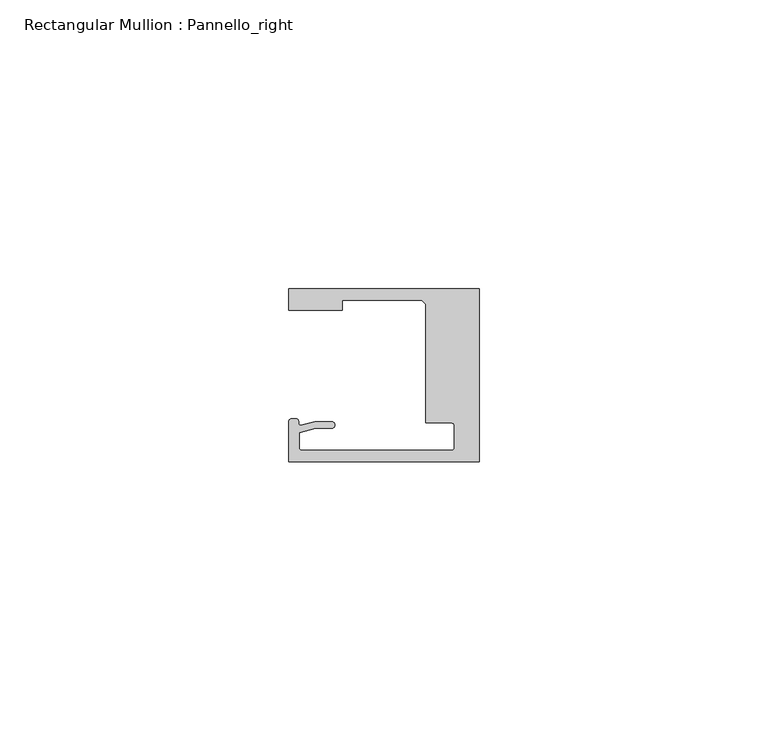
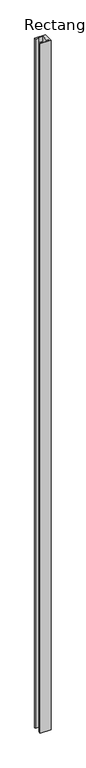
"""IFC4 building model written with IfcOpenShell, lengths in millimetres: member geometry, Rectangular Mullion : Pannello_right."""

from ifc_helpers import new_model, si_unit, frame, origin, place, context, project, spatial, polyline, circle_curve, source, transform, mapped, element, save
from ifc_brep_helpers import plane_surface, cylinder_surface, revolved_surface, extruded_surface, spline_curve, advanced_brep


def rectangular_mullion_pannello_right_fd8d7534(model_context):
    return source(origin(), model_context, "Body", "AdvancedBrep", [
        advanced_brep(
        [(-33.0, 15.0, 0.0), (-33.0, 11.3000004, 0.0), (-23.700041, 11.3000004, 0.0), (-23.700041, 13.0000004, 0.0), (-10.0000103, 13.0000004, 0.0), (-9.2999726, 12.2999849, 0.0), (-9.2999726, -8.2500595, 0.0), (-4.7999726, -8.2500595, 0.0), (-4.2999726, -8.7500595, 0.0), (-4.2999726, -12.50001, 0.0), (-4.7999726, -13.00001, 0.0), (-30.69998, -13.00001, 0.0), (-31.19998, -12.50001, 0.0), (-31.19998, -9.9657591, 0.0), (-28.3419477, -9.1999523, 0.0), (-25.59998, -9.1999523, 0.0), (-25.59998, -7.9999523, 0.0), (-28.4999305, -7.9999523, 0.0), (-30.9223017, -8.6490241, 0.0), (-33.0000135, -8.0000472, 0.0), (-33.0000135, -15.0, 0.0), (0.0, -15.0, 0.0), (0.0, 15.0, 0.0), (-33.0, 15.0, -2260.0), (0.0, 15.0, -2260.0), (0.0, -15.0, -2260.0), (-33.0000135, -15.0, -2260.0), (-33.0000135, -8.0000472, -2260.0), (-30.9223017, -8.6490241, -2260.0), (-28.4999305, -7.9999523, -2260.0), (-25.59998, -7.9999523, -2260.0), (-25.59998, -9.1999523, -2260.0), (-28.3419477, -9.1999523, -2260.0), (-31.19998, -9.9657591, -2260.0), (-31.19998, -12.50001, -2260.0), (-30.69998, -13.00001, -2260.0), (-4.7999726, -13.00001, -2260.0), (-4.2999726, -12.50001, -2260.0), (-4.2999726, -8.7500595, -2260.0), (-4.7999726, -8.2500595, -2260.0), (-9.2999726, -8.2500595, -2260.0), (-9.2999726, 12.2999849, -2260.0), (-10.0000103, 13.0000004, -2260.0), (-23.700041, 13.0000004, -2260.0), (-23.700041, 11.3000004, -2260.0), (-33.0, 11.3000004, -2260.0)],
        [
            (0, 1),
            (1, 2),
            (2, 3),
            (3, 4),
            (4, 5),
            (5, 6),
            (6, 7),
            (7, 8, circle_curve(frame((-4.7999726, -8.7500595, 0.0), z_axis=(0.0, 0.0, -1.0), x_axis=(0.0, 1.0, 0.0)), 0.5)),
            (8, 9),
            (9, 10, circle_curve(frame((-4.7999726, -12.50001, 0.0), z_axis=(0.0, 0.0, -1.0), x_axis=(1.0, 0.0, 0.0)), 0.5)),
            (10, 11),
            (11, 12, circle_curve(frame((-30.69998, -12.50001, 0.0), z_axis=(0.0, 0.0, -1.0), x_axis=(0.0, -1.0, 0.0)), 0.5)),
            (12, 13),
            (13, 14),
            (14, 15),
            (15, 16, circle_curve(frame((-25.59998, -8.5999523, 0.0), z_axis=(0.0, 0.0, 1.0), x_axis=(0.0, -1.0, 0.0)), 0.6)),
            (16, 17),
            (17, 18),
            (18, 19, spline_curve(3, [(-30.9223017, -8.6490241, 0.0), (-31.312054066, -8.717747958, 0.0), (-31.298563602, -8.366228555, 0.0), (-31.305645054, -7.690065204, 0.0), (-31.357433266, -7.563996614, 0.0), (-32.262327879, -7.456527435, 0.0), (-33.0000135, -7.457047519, 0.0), (-33.0000135, -8.0000472, 0.0)], [4, 2, 2, 4], [0.0, 0.001840817752199412, 0.004996616814974408, 0.007702013405570312])),
            (19, 20),
            (20, 21),
            (21, 22),
            (22, 0),
            (23, 24),
            (24, 25),
            (25, 26),
            (26, 27),
            (27, 28, spline_curve(3, [(-33.0000135, -8.0000472, -2260.0), (-33.0000135, -7.457047519, -2260.0), (-32.262327879, -7.456527435, -2260.0), (-31.357433266, -7.563996614, -2260.0), (-31.305645054, -7.690065204, -2260.0), (-31.298563602, -8.366228555, -2260.0), (-31.312054066, -8.717747958, -2260.0), (-30.9223017, -8.6490241, -2260.0)], [4, 2, 2, 4], [0.0, 0.0027053965905959043, 0.0058611956533709, 0.007702013405570312])),
            (28, 29),
            (29, 30),
            (30, 31, circle_curve(frame((-25.59998, -8.5999523, -2260.0), z_axis=(0.0, 0.0, -1.0), x_axis=(0.0, -1.0, 0.0)), 0.6)),
            (31, 32),
            (32, 33),
            (33, 34),
            (34, 35, circle_curve(frame((-30.69998, -12.50001, -2260.0), z_axis=(0.0, 0.0, 1.0), x_axis=(0.0, -1.0, 0.0)), 0.5)),
            (35, 36),
            (36, 37, circle_curve(frame((-4.7999726, -12.50001, -2260.0), z_axis=(0.0, 0.0, 1.0), x_axis=(1.0, 0.0, 0.0)), 0.5)),
            (37, 38),
            (38, 39, circle_curve(frame((-4.7999726, -8.7500595, -2260.0), z_axis=(0.0, 0.0, 1.0), x_axis=(0.0, 1.0, 0.0)), 0.5)),
            (39, 40),
            (40, 41),
            (41, 42),
            (42, 43),
            (43, 44),
            (44, 45),
            (45, 23),
            (0, 23),
            (45, 1),
            (44, 2),
            (43, 3),
            (42, 4),
            (41, 5),
            (40, 6),
            (39, 7),
            (38, 8),
            (37, 9),
            (36, 10),
            (35, 11),
            (34, 12),
            (33, 13),
            (32, 14),
            (31, 15),
            (30, 16),
            (29, 17),
            (28, 18),
            (27, 19),
            (26, 20),
            (25, 21),
            (24, 22),
        ],
        [
            plane_surface(frame((0.0, -36.2491502, 0.0), z_axis=(0.0, 0.0, 1.0), x_axis=(-1.0, 0.0, 0.0))),
            plane_surface(frame((0.0, -36.2491502, -2260.0), z_axis=(0.0, 0.0, -1.0), x_axis=(-1.0, 0.0, 0.0))),
            plane_surface(frame((-33.0, 15.0, 0.0), z_axis=(-1.0, 0.0, 0.0), x_axis=(0.0, 0.0, -1.0))),
            plane_surface(frame((-33.0, 11.3000004, 0.0), z_axis=(0.0, -1.0, 0.0), x_axis=(0.0, 0.0, -1.0))),
            plane_surface(frame((-23.700041, 11.3000004, 0.0), z_axis=(1.0, 0.0, 0.0), x_axis=(0.0, 0.0, -1.0))),
            plane_surface(frame((-23.700041, 13.0000004, 0.0), z_axis=(0.0, -1.0, 0.0), x_axis=(0.0, 0.0, -1.0))),
            plane_surface(frame((-10.0000103, 13.0000004, 0.0), z_axis=(-0.7070955486278075, -0.7071180135668587, 0.0), x_axis=(0.0, 0.0, -1.0))),
            plane_surface(frame((-9.2999726, 12.2999849, 0.0), z_axis=(-1.0, 0.0, 0.0), x_axis=(0.0, 0.0, -1.0))),
            plane_surface(frame((-9.2999726, -8.2500595, 0.0), z_axis=(0.0, -1.0, 0.0), x_axis=(0.0, 0.0, -1.0))),
            revolved_surface(polyline([(-4.7999726, -8.2500595, -2260.0), (-4.7999726, -8.2500595, 0.0)]), (-4.7999726, -8.7500595, 0.0), (0.0, 0.0, -1.0)),
            plane_surface(frame((-4.2999726, -8.7500595, 0.0), z_axis=(-1.0, 0.0, 0.0), x_axis=(0.0, 0.0, -1.0))),
            revolved_surface(polyline([(-4.2999726, -12.50001, -2260.0), (-4.2999726, -12.50001, 0.0)]), (-4.7999726, -12.50001, 0.0), (0.0, 0.0, -1.0)),
            plane_surface(frame((-4.7999726, -13.00001, 0.0), z_axis=(0.0, 1.0, 0.0), x_axis=(0.0, 0.0, -1.0))),
            revolved_surface(polyline([(-30.69998, -13.00001, -2260.0), (-30.69998, -13.00001, 0.0)]), (-30.69998, -12.50001, 0.0), (0.0, 0.0, -1.0)),
            plane_surface(frame((-31.19998, -12.50001, 0.0), z_axis=(1.0, 0.0, 0.0), x_axis=(0.0, 0.0, -1.0))),
            plane_surface(frame((-31.19998, -9.9657591, 0.0), z_axis=(0.2588188320428738, -0.9659258833782035, 0.0), x_axis=(0.0, 0.0, -1.0))),
            plane_surface(frame((-28.3419477, -9.1999523, 0.0), z_axis=(0.0, -1.0, 0.0), x_axis=(0.0, 0.0, -1.0))),
            cylinder_surface(frame((-25.59998, -8.5999523, 0.0), z_axis=(0.0, 0.0, 1.0), x_axis=(0.0, -1.0, 0.0)), 0.6),
            plane_surface(frame((-25.59998, -7.9999523, 0.0), z_axis=(0.0, 1.0, 0.0), x_axis=(0.0, 0.0, -1.0))),
            plane_surface(frame((-28.4999305, -7.9999523, 0.0), z_axis=(-0.2588188320019168, 0.965925883389178, 0.0), x_axis=(0.0, 0.0, -1.0))),
            extruded_surface(spline_curve(3, [(-30.9223017, -8.6490241, -2260.0), (-31.312054066, -8.717747958, -2260.0), (-31.298563602, -8.366228555, -2260.0), (-31.305645054, -7.690065204, -2260.0), (-31.357433266, -7.563996614, -2260.0), (-32.262327879, -7.456527435, -2260.0), (-33.0000135, -7.457047519, -2260.0), (-33.0000135, -8.0000472, -2260.0)], [4, 2, 2, 4], [0.0, 0.001840817752199412, 0.004996616814974408, 0.007702013405570312]), (0.0, 0.0, 2260.0), 2260.0),
            plane_surface(frame((-33.0000135, -8.0000472, 0.0), z_axis=(-1.0, 0.0, 0.0), x_axis=(0.0, 0.0, -1.0))),
            plane_surface(frame((-33.0000135, -15.0, 0.0), z_axis=(0.0, -1.0, 0.0), x_axis=(0.0, 0.0, -1.0))),
            plane_surface(frame((0.0, -15.0, 0.0), z_axis=(1.0, 0.0, 0.0), x_axis=(0.0, 0.0, -1.0))),
            plane_surface(frame((0.0, 15.0, 0.0), z_axis=(0.0, 1.0, 0.0), x_axis=(0.0, 0.0, -1.0))),
        ],
        [
            (0, [[1, 2, 3, 4, 5, 6, 7, 8, 9, 10, 11, 12, 13, 14, 15, 16, 17, 18, 19, 20, 21, 22, 23]]),
            (1, [[24, 25, 26, 27, 28, 29, 30, 31, 32, 33, 34, 35, 36, 37, 38, 39, 40, 41, 42, 43, 44, 45, 46]]),
            (2, [[-1, 47, -46, 48]]),
            (3, [[-2, -48, -45, 49]]),
            (4, [[-3, -49, -44, 50]]),
            (5, [[-4, -50, -43, 51]]),
            (6, [[-5, -51, -42, 52]]),
            (7, [[-6, -52, -41, 53]]),
            (8, [[-7, -53, -40, 54]]),
            (9, [[-8, -54, -39, 55]]),
            (10, [[-9, -55, -38, 56]]),
            (11, [[-10, -56, -37, 57]]),
            (12, [[-11, -57, -36, 58]]),
            (13, [[-12, -58, -35, 59]]),
            (14, [[-13, -59, -34, 60]]),
            (15, [[-14, -60, -33, 61]]),
            (16, [[-15, -61, -32, 62]]),
            (17, [[-16, -62, -31, 63]]),
            (18, [[-17, -63, -30, 64]]),
            (19, [[-18, -64, -29, 65]]),
            (20, [[-19, -65, -28, 66]]),
            (21, [[-20, -66, -27, 67]]),
            (22, [[-21, -67, -26, 68]]),
            (23, [[-22, -68, -25, 69]]),
            (24, [[-23, -69, -24, -47]]),
        ],
    ),
    ])


if __name__ == "__main__":
    model = new_model("IFC4")
    model_context = context("Model", 3, world=origin())
    ifc_project = project(units=[si_unit("LENGTHUNIT", "METRE", prefix="MILLI")], contexts=[model_context])
    site = spatial("IfcSite", under=ifc_project)
    building = spatial("IfcBuilding", under=site)
    placement = place(None, origin())
    rectangular_mullion_pannello_right_shape = rectangular_mullion_pannello_right_fd8d7534(model_context)
    element("IfcMember", 1, ObjectType="Rectangular Mullion : Pannello_right", at=placement, inside=building, context=model_context, shape_type="MappedRepresentation", body=[
        mapped(rectangular_mullion_pannello_right_shape, transform((0.0, 0.0, 0.0), x_axis=(1.0, 0.0, 0.0), y_axis=(0.0, 1.0, 0.0), z_axis=(0.0, 0.0, 1.0))),
    ])
    save(model, "model.ifc")

# Revit data of these elements
# Type "Rectangular Mullion : Pannello_right"
#   built-in parameter 1007322 = 0.0984252 (stored number, unit not read)
#   built-in parameter 1007321 = 0.0305117 (stored number, unit not read)
#   built-in parameter 1007320 = 0 (stored number, unit not read)
